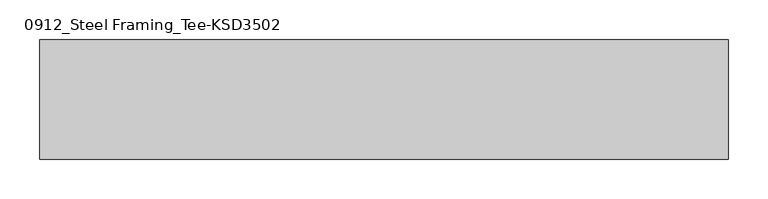
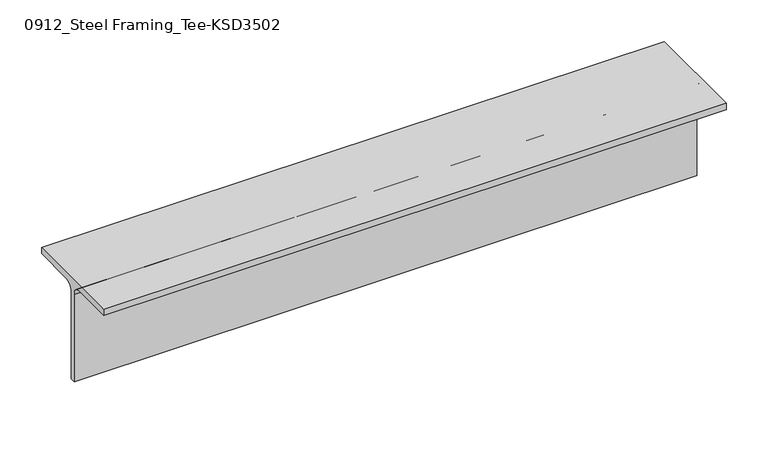
"""IFC4 building model written with IfcOpenShell, lengths in millimetres: member geometry, 0912_Steel Framing_Tee-KSD3502 : H_SB_ASB_CT-150x150x6.5x9."""

from ifc_helpers import new_model, si_unit, point, frame, frame_2d, origin, place, context, project, spatial, polyline, circle_curve, trimmed, segment, composite_curve, outline, extrude, source, transform, mapped, element, save


def member_0912_steel_framing_tee_ksd3502_f1b537a8(model_context):
    return source(origin(), model_context, "Body", "SweptSolid", [
        extrude(outline(composite_curve([segment(polyline([(-75.0, 75.0), (75.0, 75.0), (75.0, 66.0), (16.25, 66.0)]), True, "CONTINUOUS"), segment(trimmed(circle_curve(frame_2d((16.25, 53.0)), 13.0), [point((16.25, 66.0))], [point((3.25, 53.0))], True, "CARTESIAN"), True, "CONTINUOUS"), segment(polyline([(3.25, 53.0), (3.25, -75.0), (-3.25, -75.0), (-3.25, 53.0)]), True, "CONTINUOUS"), segment(trimmed(circle_curve(frame_2d((-16.25, 53.0)), 13.0), [point((-3.25, 53.0))], [point((-16.25, 66.0))], True, "CARTESIAN"), True, "CONTINUOUS"), segment(polyline([(-16.25, 66.0), (-75.0, 66.0), (-75.0, 75.0)]), True, "CONTINUOUS")], self_intersect=False)), frame((-500.0, 0.0, 0.0), z_axis=(1.0, 0.0, 0.0), x_axis=(0.0, 1.0, 0.0)), (0.0, 0.0, 1.0), 865.9),
    ])


if __name__ == "__main__":
    model = new_model("IFC4")
    model_context = context("Model", 3, world=origin())
    ifc_project = project(units=[si_unit("LENGTHUNIT", "METRE", prefix="MILLI")], contexts=[model_context])
    site = spatial("IfcSite", under=ifc_project)
    building = spatial("IfcBuilding", under=site)
    placement = place(None, origin())
    member_0912_steel_framing_tee_ksd3502_shape = member_0912_steel_framing_tee_ksd3502_f1b537a8(model_context)
    element("IfcMember", 1, ObjectType="0912_Steel Framing_Tee-KSD3502 : H_SB_ASB_CT-150x150x6.5x9", at=placement, inside=building, context=model_context, shape_type="MappedRepresentation", body=[
        mapped(member_0912_steel_framing_tee_ksd3502_shape, transform((0.0, 0.0, 0.0), x_axis=(1.0, 0.0, 0.0), y_axis=(0.0, 1.0, 0.0), z_axis=(0.0, 0.0, 1.0))),
    ])
    save(model, "model.ifc")

# Revit data of these elements
# Type "0912_Steel Framing_Tee-KSD3502 : H_SB_ASB_CT-150x150x6.5x9"
#   H_WM Code_1 = "S01AA003-00001 | Main Steel Structure Fabrication Work | Shelter/Building | Light Steel - Standard (30KG/M>Weight) | Material: (   )"
#   H_WM Code_2 = "S03AA029-00001 | Main Steel Structure Erection Work | Shelter/Building | Light Steel (30KG/M>Weight) | Material: (   )"
#   H_WM Code_3 = "S01AA010-00001 | Main Steel Structure Fabrication Work | Shelter/Building | Steel Painting/Coating | for Non-Fireproofed Steel Surface, Surface Preparation, Primer, Second & Final Coat | Material: (   )"
#   H_Q'ty Cal Type Tag = "SB-Q2"
#   Width = 15.0 cm
#   Web Thickness = 0.65 cm
#   Web Fillet = 1.3 cm
#   Section Area = 23.39 cm²
#   Perimeter = 0.60 m²/m
#   Nominal Weight = 18.40 kgf/m
#   Height = 15.0 cm
#   Flange Thickness = 0.9 cm
#   Centroid Vertical = 7.5 cm
#   Centroid Horizontal = 7.5 cm
#   Length [instance default] = 1.5000 m
#   Structural Material [instance default] = Steel, 45-345
#   Warping Constant = (empty or 0)
#   Torsional Moment of Inertia = 0
#   Section Name Key = ""
#   Plastic Modulus weak axis = 0
#   Plastic Modulus strong axis = 0
#   Moment of Inertia weak axis = 0
#   Moment of Inertia strong axis = 0
#   Elastic Modulus weak axis = 0
#   Elastic Modulus strong axis = 0
#   Bolt Spacing = 0
#   Assembly Code = ""
# Element 1 (IfcMember, "0912_Steel Framing_Tee-KSD3502 : H_SB_ASB_CT-150x150x6.5x9")
#   Structural Material = none
# Materials
#   "Steel, 45-345": class "Metal", colour RGB 189 187 185, transparency 0, Description = "Steel 345 MPa", Cost = 0
